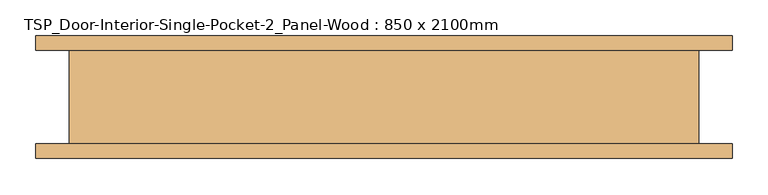
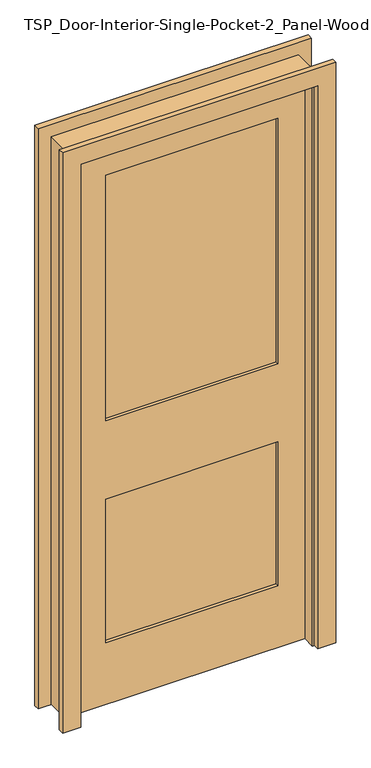
"""IFC4 building model written with IfcOpenShell, lengths in millimetres: door geometry, TSP_Door-Interior-Single-Pocket-2_Panel-Wood : 850 x 2100mm."""

from ifc_helpers import new_model, si_unit, frame, origin, place, context, project, spatial, polyline, outline, extrude, faceted_brep, source, transform, mapped, element, save


def tsp_door_interior_single_pocket_2_panel_wood_850_x_2100mm_8f7b9fad(model_context):
    return source(origin(), model_context, "Body", "SolidModel", [
        extrude(outline(polyline([(0.0, 405.95), (0.0, 470.95), (2171.35, 470.95), (2171.35, -496.35), (0.0, -496.35), (0.0, -431.35), (2106.35, -431.35), (2106.35, 405.95), (0.0, 405.95)])), frame((0.0, 65.0, 0.0), z_axis=(0.0, 1.0, 0.0), x_axis=(0.0, 0.0, 1.0)), (0.0, 0.0, 1.0), 20.0),
        extrude(outline(polyline([(0.0, 405.95), (0.0, 470.95), (2171.35, 470.95), (2171.35, -496.35), (0.0, -496.35), (0.0, -431.35), (2106.35, -431.35), (2106.35, 405.95), (0.0, 405.95)])), frame((0.0, -85.0, 0.0), z_axis=(0.0, 1.0, 0.0), x_axis=(0.0, 0.0, 1.0)), (0.0, 0.0, 1.0), 20.0),
        extrude(outline(polyline([(2100.0, -425.4), (0.0, -425.4), (0.0, 424.6), (2100.0, 424.6), (2100.0, -425.4)]), holes=[polyline([(1980.0, -305.4), (1980.0, 304.6), (1060.45, 304.6), (1060.45, -305.4), (1980.0, -305.4)]), polyline([(768.35, -305.4), (768.35, 304.6), (230.0, 304.6), (230.0, -305.4), (768.35, -305.4)])]), frame((0.0, -17.5, 0.0), z_axis=(0.0, 1.0, 0.0), x_axis=(0.0, 0.0, 1.0)), (0.0, 0.0, 1.0), 35.0),
        extrude(outline(polyline([(304.6, -5.8333333), (-305.4, -5.8333333), (-305.4, 5.8333333), (304.6, 5.8333333), (304.6, -5.8333333)])), frame((0.0, 0.0, 1060.45), z_axis=(0.0, 0.0, 1.0), x_axis=(1.0, 0.0, 0.0)), (0.0, 0.0, 1.0), 919.55),
        extrude(outline(polyline([(304.6, -5.8333333), (-305.4, -5.8333333), (-305.4, 5.8333333), (304.6, 5.8333333), (304.6, -5.8333333)])), frame((0.0, 0.0, 230.0), z_axis=(0.0, 0.0, 1.0), x_axis=(1.0, 0.0, 0.0)), (0.0, 0.0, 1.0), 538.35),
        faceted_brep([(425.0, -65.0, 0.0), (425.0, -17.5, 0.0), (425.0, -17.5, 2100.0), (425.0, 17.5, 2100.0), (425.0, 17.5, 0.0), (425.0, 65.0, 0.0), (425.0, 65.0, 2125.4), (425.0, -65.0, 2125.4), (-450.4, -65.0, 2125.4), (-450.4, -65.0, 0.0), (-425.0, -65.0, 0.0), (-425.0, -65.0, 2100.0), (399.6, -65.0, 2100.0), (399.6, -65.0, 0.0), (-425.0, 65.0, 2100.0), (399.6, 65.0, 2100.0), (399.6, 17.5, 2100.0), (399.6, -17.5, 2100.0), (399.6, 65.0, 0.0), (-425.0, 65.0, 0.0), (-450.4, 65.0, 0.0), (-450.4, 65.0, 2125.4), (399.6, -17.5, 0.0), (399.6, 17.5, 0.0)], [[[0, 1, 2, 3, 4, 5, 6, 7]], [[0, 7, 8, 9, 10, 11, 12, 13]], [[11, 14, 15, 16, 3, 2, 17, 12]], [[6, 5, 18, 15, 14, 19, 20, 21]], [[6, 21, 8, 7]], [[10, 9, 20, 19]], [[11, 10, 19, 14]], [[9, 8, 21, 20]], [[1, 0, 13, 22]], [[5, 4, 23, 18]], [[18, 23, 16, 15]], [[23, 4, 3, 16]], [[1, 22, 17, 2]], [[22, 13, 12, 17]]]),
    ])


if __name__ == "__main__":
    model = new_model("IFC4")
    model_context = context("Model", 3, world=origin())
    ifc_project = project(units=[si_unit("LENGTHUNIT", "METRE", prefix="MILLI")], contexts=[model_context])
    site = spatial("IfcSite", under=ifc_project)
    building = spatial("IfcBuilding", under=site)
    placement = place(None, origin())
    tsp_door_interior_single_pocket_2_panel_wood_850_x_2100mm_shape = tsp_door_interior_single_pocket_2_panel_wood_850_x_2100mm_8f7b9fad(model_context)
    element("IfcDoor", 1, ObjectType="TSP_Door-Interior-Single-Pocket-2_Panel-Wood : 850 x 2100mm", at=placement, inside=building, context=model_context, shape_type="MappedRepresentation", body=[
        mapped(tsp_door_interior_single_pocket_2_panel_wood_850_x_2100mm_shape, transform((0.0, 0.0, 0.0), x_axis=(1.0, 0.0, 0.0), y_axis=(0.0, 1.0, 0.0), z_axis=(0.0, 0.0, 1.0))),
    ])
    save(model, "model.ifc")

# Revit data of these elements
# Type "TSP_Door-Interior-Single-Pocket-2_Panel-Wood : 850 x 2100mm"
#   Model = "TSP_DOOR02W"
#   Type Mark = "417"
#   Assembly Code = "C1020300"
#   Analytic Construction = "Wooden"
#   Top Rail = 120 mm
#   Thickness = 35 mm
#   Thermal Resistance (R) = 0.455703 (m²·K)/W
#   Stiles = 120 mm
#   Rough Width = 1725 mm
#   Rough Height = 2215 mm
#   Lock Rail = 120 mm
#   Location [instance default] = 850 mm
#   Height = 2100 mm
#   Width = 850 mm
#   Heat Transfer Coefficient (U) = 2.19465 W/(m²·K)
#   Bottom Rail = 230 mm
#   Panel Open [instance default] = no
#   Trim Material = Cherry
#   Panel Material = Cherry
#   Frame Material = Cherry
#   Visual Light Transmittance = 0
#   Solar Heat Gain Coefficient = 0
#   Wall Closure = (empty or 0)
#   Function = (empty or 0)
# Element 1 (IfcDoor, "TSP_Door-Interior-Single-Pocket-2_Panel-Wood : 850 x 2100mm")
#   Materials on its faces: "Cherry"
# Materials
#   "Cherry": class "Wood", colour RGB 226 177 128, transparency 0, Description = "Prunus Serotina", Cost = 0
